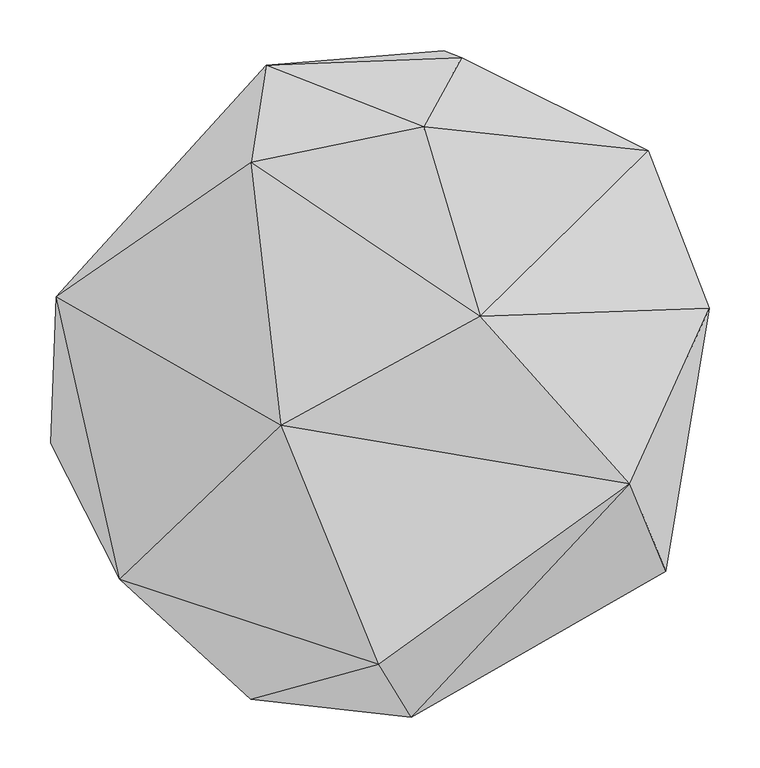
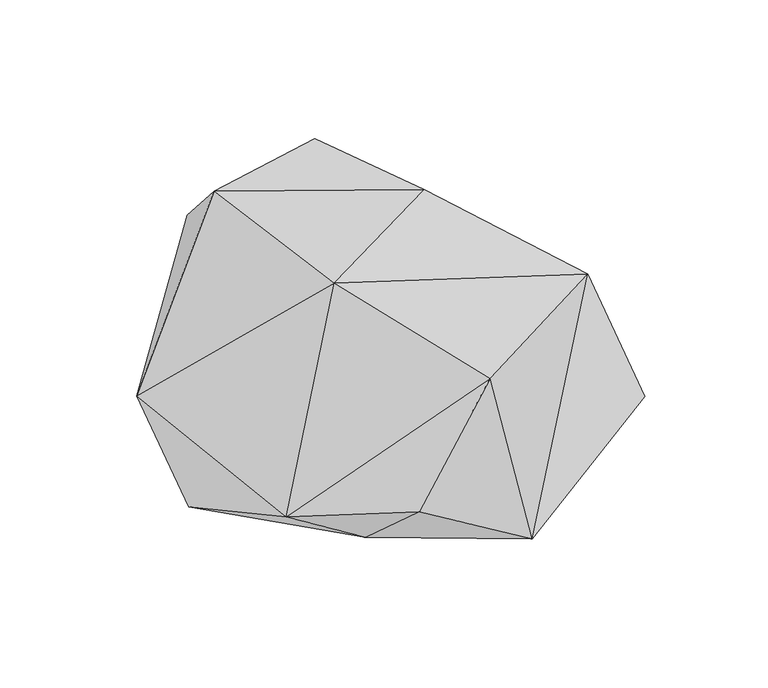
"""IFC4 building model written with IfcOpenShell, lengths in millimetres: geographic element geometry, Enscape AssetDefinition - Bush 067 Blue Fescue : Enscape AssetDefinition - Bush 067 Blue Fescue."""

from ifc_helpers import new_model, si_unit, origin, place, context, project, spatial, faceted_brep, source, transform, mapped, element, save


def geographic_element_765c0492(model_context):
    return source(origin(), model_context, "Body", "Brep", [
        faceted_brep([(251.1489987, 226.5100032, 60.7430004), (311.033994, 70.9460005, 118.4879988), (289.8010015, -2.749, 24.0529999), (268.0009902, -188.9420003, 97.1650034), (232.8229994, -102.6019976, 250.6119907), (84.7430006, 63.1560013, 335.4850113), (154.945001, -125.0769943, -0.359), (116.3270026, 116.6080013, 0.0), (16.9009995, -333.2819939, 48.1190011), (-15.1899997, -280.7500064, 280.4259956), (-111.8260026, -44.7070003, 321.9749928), (-141.5710002, 215.2640074, 319.8809922), (29.2249992, 250.3719926, 322.0750093), (-271.4389861, -196.7149973, 100.6689966), (-333.8690102, 82.4719965, 144.0880001), (-141.6420043, -315.1260018, 134.7180009), (-133.7900013, -163.308993, -0.029), (-339.6469951, -62.2249991, 59.1700003), (-206.0219944, 63.9680028, -0.016), (-197.8230029, 229.3030024, 55.6700006), (-126.4279932, 311.1569881, 218.8390046), (48.6560017, 325.5510032, 59.5199987), (66.7610019, 318.4059858, 202.3009956), (-76.4829963, 156.1460048, -1.7509999)], [[[0, 1, 2]], [[1, 3, 2]], [[4, 3, 1]], [[4, 1, 5]], [[1, 0, 5]], [[2, 3, 6]], [[2, 6, 7]], [[2, 7, 0]], [[8, 3, 4]], [[3, 8, 6]], [[9, 8, 4]], [[10, 4, 5]], [[9, 4, 10]], [[11, 5, 12]], [[10, 5, 11]], [[12, 5, 0]], [[13, 9, 10]], [[10, 11, 14]], [[10, 14, 13]], [[13, 15, 9]], [[15, 8, 9]], [[8, 15, 16]], [[6, 8, 16]], [[15, 13, 16]], [[14, 17, 13]], [[17, 16, 13]], [[14, 18, 17]], [[19, 18, 14]], [[14, 11, 20]], [[20, 19, 14]], [[12, 20, 11]], [[21, 19, 20]], [[12, 22, 20]], [[21, 20, 22]], [[19, 23, 18]], [[19, 21, 23]], [[18, 23, 6]], [[17, 18, 16]], [[16, 18, 6]], [[23, 21, 7]], [[7, 6, 23]], [[21, 0, 7]], [[22, 0, 21]], [[12, 0, 22]]]),
    ])


if __name__ == "__main__":
    model = new_model("IFC4")
    model_context = context("Model", 3, world=origin())
    ifc_project = project(units=[si_unit("LENGTHUNIT", "METRE", prefix="MILLI")], contexts=[model_context])
    site = spatial("IfcSite", under=ifc_project)
    building = spatial("IfcBuilding", under=site)
    placement = place(None, origin())
    geographic_element_shape = geographic_element_765c0492(model_context)
    element("IfcGeographicElement", 1, ObjectType="Enscape AssetDefinition - Bush 067 Blue Fescue : Enscape AssetDefinition - Bush 067 Blue Fescue", at=placement, inside=building, context=model_context, shape_type="MappedRepresentation", body=[
        mapped(geographic_element_shape, transform((0.0, 0.0, 0.0), x_axis=(1.0, 0.0, 0.0), y_axis=(0.0, 1.0, 0.0), z_axis=(0.0, 0.0, 1.0))),
    ])
    save(model, "model.ifc")

# Revit data of these elements
# Type "Enscape AssetDefinition - Bush 067 Blue Fescue : Enscape AssetDefinition - Bush 067 Blue Fescue"
#   EnscapeAssetSource = "REMOTE"
#   EnscapeAssetId = "0cf11ac6-b57d-4a71-bc34-b1c1f1ddb68a"
#   Height = 0.335485 m
#   EnscapeNativeAssetHeight = 0.335485 m
#   Default Elevation = 0
